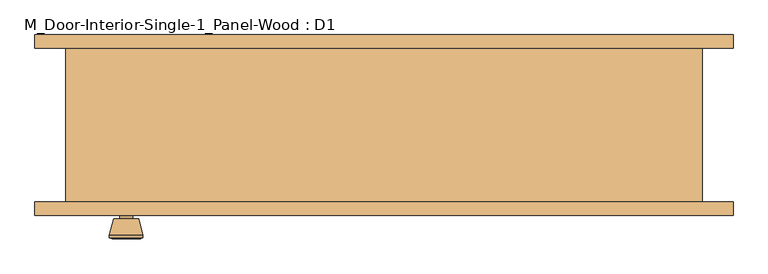
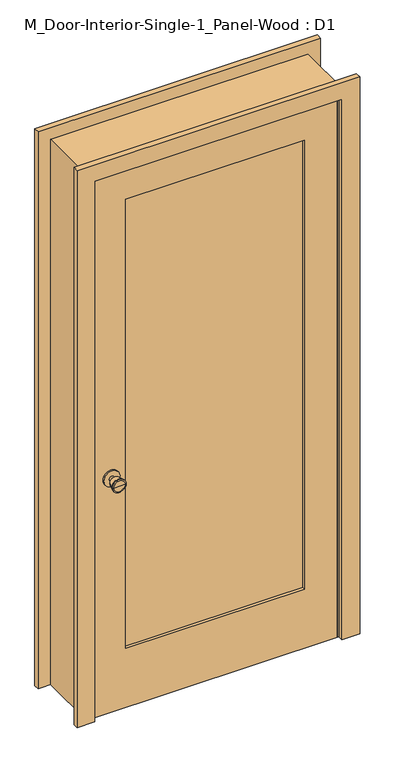
"""IFC4 building model written with IfcOpenShell, lengths in millimetres: door geometry, M_Door-Interior-Single-1_Panel-Wood : D1."""

from ifc_helpers import new_model, si_unit, point, frame, frame_2d, origin, place, context, project, spatial, polyline, circle_curve, trimmed, segment, composite_curve, outline, extrude, faceted_brep, source, transform, mapped, element, save
from ifc_brep_helpers import plane_surface, cylinder_surface, revolved_surface, advanced_brep


def m_door_interior_single_1_panel_wood_d1_ac8a812a(model_context):
    return source(origin(), model_context, "Body", "SolidModel", [
        advanced_brep(
        [(-385.0, -70.825, 914.4), (-395.0, -70.825, 914.4), (-375.0, -70.825, 914.4), (-364.5241324, -21.825, 914.4), (-405.4758676, -21.825, 914.4), (-385.0, -21.825, 914.4), (-360.0, -23.6528681, 914.4), (-410.0, -23.6528681, 914.4), (-360.0, -27.1165463, 914.4), (-410.0, -27.1165463, 914.4), (-366.363764, -51.825, 914.4), (-403.636236, -51.825, 914.4), (-375.0, -51.825, 914.4), (-395.0, -51.825, 914.4)],
        [
            (0, 1),
            (1, 2, circle_curve(frame((-385.0, -70.825, 914.4), z_axis=(0.0, -1.0, 0.0), x_axis=(-1.0, 0.0, 0.0)), 10.0)),
            (2, 0),
            (2, 1, circle_curve(frame((-385.0, -70.825, 914.4), z_axis=(0.0, -1.0, 0.0), x_axis=(-1.0, 0.0, 0.0)), 10.0)),
            (3, 4, circle_curve(frame((-385.0, -21.825, 914.4), z_axis=(0.0, 1.0, 0.0), x_axis=(-1.0, 0.0, 0.0)), 20.4758676)),
            (4, 5),
            (5, 3),
            (4, 3, circle_curve(frame((-385.0, -21.825, 914.4), z_axis=(0.0, 1.0, 0.0), x_axis=(-1.0, 0.0, 0.0)), 20.4758676)),
            (6, 7, circle_curve(frame((-385.0, -23.6528681, 914.4), z_axis=(0.0, 1.0, 0.0), x_axis=(-1.0, 0.0, 0.0)), 25.0)),
            (7, 4),
            (3, 6),
            (7, 6, circle_curve(frame((-385.0, -23.6528681, 914.4), z_axis=(0.0, 1.0, 0.0), x_axis=(-1.0, 0.0, 0.0)), 25.0)),
            (8, 9, circle_curve(frame((-385.0, -27.1165463, 914.4), z_axis=(0.0, 1.0, 0.0), x_axis=(-1.0, 0.0, 0.0)), 25.0)),
            (9, 7),
            (6, 8),
            (9, 8, circle_curve(frame((-385.0, -27.1165463, 914.4), z_axis=(0.0, 1.0, 0.0), x_axis=(-1.0, 0.0, 0.0)), 25.0)),
            (10, 11, circle_curve(frame((-385.0, -51.825, 914.4), z_axis=(0.0, 1.0, 0.0), x_axis=(-1.0, 0.0, 0.0)), 18.636236)),
            (11, 9),
            (8, 10),
            (11, 10, circle_curve(frame((-385.0, -51.825, 914.4), z_axis=(0.0, 1.0, 0.0), x_axis=(-1.0, 0.0, 0.0)), 18.636236)),
            (12, 13, circle_curve(frame((-385.0, -51.825, 914.4), z_axis=(0.0, 1.0, 0.0), x_axis=(-1.0, 0.0, 0.0)), 10.0)),
            (13, 11),
            (10, 12),
            (13, 12, circle_curve(frame((-385.0, -51.825, 914.4), z_axis=(0.0, 1.0, 0.0), x_axis=(-1.0, 0.0, 0.0)), 10.0)),
            (1, 13),
            (12, 2),
        ],
        [
            plane_surface(frame((-385.0, -70.825, 914.4), z_axis=(0.0, -1.0, 0.0), x_axis=(-1.0, 0.0, 0.0))),
            plane_surface(frame((-385.0, -21.825, 914.4), z_axis=(0.0, 1.0, 0.0), x_axis=(-1.0, 0.0, 0.0))),
            revolved_surface(polyline([(-405.4758676, -21.825, 914.4), (-410.0, -23.6528681, 914.4)]), (-385.0, -70.825, 914.4), (0.0, -1.0, 0.0)),
            cylinder_surface(frame((-385.0, -70.825, 914.4), z_axis=(0.0, -1.0, 0.0), x_axis=(-1.0, 0.0, 0.0)), 25.0),
            revolved_surface(polyline([(-410.0, -27.1165463, 914.4), (-403.636236, -51.825, 914.4)]), (-385.0, -70.825, 914.4), (0.0, -1.0, 0.0)),
            plane_surface(frame((-385.0, -51.825, 914.4), z_axis=(0.0, -1.0, 0.0), x_axis=(-1.0, 0.0, 0.0))),
            cylinder_surface(frame((-385.0, -70.825, 914.4), z_axis=(0.0, -1.0, 0.0), x_axis=(-1.0, 0.0, 0.0)), 10.0),
        ],
        [
            (0, [[1, 2, 3]]),
            (0, [[-3, 4, -1]]),
            (1, [[5, 6, 7]]),
            (1, [[8, -7, -6]]),
            (2, [[9, 10, -5, 11]]),
            (2, [[12, -11, -8, -10]]),
            (3, [[13, 14, -9, 15]]),
            (3, [[16, -15, -12, -14]]),
            (4, [[17, 18, -13, 19]]),
            (4, [[20, -19, -16, -18]]),
            (5, [[21, 22, -17, 23]]),
            (5, [[24, -23, -20, -22]]),
            (6, [[-2, 25, -21, 26]]),
            (6, [[-4, -26, -24, -25]]),
        ],
    ),
        extrude(outline(composite_curve([segment(trimmed(circle_curve(frame_2d((914.4, -385.0)), 30.0), [point((914.4, -415.0))], [point((914.4, -355.0))], False, "CARTESIAN"), True, "CONTINUOUS"), segment(trimmed(circle_curve(frame_2d((914.4, -385.0)), 30.0), [point((914.4, -355.0))], [point((914.4, -415.0))], False, "CARTESIAN"), True, "CONTINUOUS")], self_intersect=False)), frame((0.0, -76.825, 0.0), z_axis=(0.0, 1.0, 0.0), x_axis=(0.0, 0.0, 1.0)), (0.0, 0.0, 1.0), 6.0),
        advanced_brep(
        [(-385.0, -117.825, 914.4), (-375.0, -117.825, 914.4), (-395.0, -117.825, 914.4), (-364.5241324, -166.825, 914.4), (-385.0, -166.825, 914.4), (-405.4758676, -166.825, 914.4), (-360.0, -164.9971319, 914.4), (-410.0, -164.9971319, 914.4), (-360.0, -161.5334537, 914.4), (-410.0, -161.5334537, 914.4), (-366.363764, -136.825, 914.4), (-403.636236, -136.825, 914.4), (-375.0, -136.825, 914.4), (-395.0, -136.825, 914.4)],
        [
            (0, 1),
            (1, 2, circle_curve(frame((-385.0, -117.825, 914.4), z_axis=(0.0, 1.0, 0.0), x_axis=(-1.0, 0.0, 0.0)), 10.0)),
            (2, 0),
            (2, 1, circle_curve(frame((-385.0, -117.825, 914.4), z_axis=(0.0, 1.0, 0.0), x_axis=(-1.0, 0.0, 0.0)), 10.0)),
            (3, 4),
            (4, 5),
            (5, 3, circle_curve(frame((-385.0, -166.825, 914.4), z_axis=(0.0, -1.0, 0.0), x_axis=(-1.0, 0.0, 0.0)), 20.4758676)),
            (3, 5, circle_curve(frame((-385.0, -166.825, 914.4), z_axis=(0.0, -1.0, 0.0), x_axis=(-1.0, 0.0, 0.0)), 20.4758676)),
            (6, 3),
            (5, 7),
            (7, 6, circle_curve(frame((-385.0, -164.9971319, 914.4), z_axis=(0.0, -1.0, 0.0), x_axis=(-1.0, 0.0, 0.0)), 25.0)),
            (6, 7, circle_curve(frame((-385.0, -164.9971319, 914.4), z_axis=(0.0, -1.0, 0.0), x_axis=(-1.0, 0.0, 0.0)), 25.0)),
            (8, 6),
            (7, 9),
            (9, 8, circle_curve(frame((-385.0, -161.5334537, 914.4), z_axis=(0.0, -1.0, 0.0), x_axis=(-1.0, 0.0, 0.0)), 25.0)),
            (8, 9, circle_curve(frame((-385.0, -161.5334537, 914.4), z_axis=(0.0, -1.0, 0.0), x_axis=(-1.0, 0.0, 0.0)), 25.0)),
            (10, 8),
            (9, 11),
            (11, 10, circle_curve(frame((-385.0, -136.825, 914.4), z_axis=(0.0, -1.0, 0.0), x_axis=(-1.0, 0.0, 0.0)), 18.636236)),
            (10, 11, circle_curve(frame((-385.0, -136.825, 914.4), z_axis=(0.0, -1.0, 0.0), x_axis=(-1.0, 0.0, 0.0)), 18.636236)),
            (12, 10),
            (11, 13),
            (13, 12, circle_curve(frame((-385.0, -136.825, 914.4), z_axis=(0.0, -1.0, 0.0), x_axis=(-1.0, 0.0, 0.0)), 10.0)),
            (12, 13, circle_curve(frame((-385.0, -136.825, 914.4), z_axis=(0.0, -1.0, 0.0), x_axis=(-1.0, 0.0, 0.0)), 10.0)),
            (1, 12),
            (13, 2),
        ],
        [
            plane_surface(frame((-385.0, -117.825, 914.4), z_axis=(0.0, 1.0, 0.0), x_axis=(-1.0, 0.0, 0.0))),
            plane_surface(frame((-385.0, -166.825, 914.4), z_axis=(0.0, -1.0, 0.0), x_axis=(-1.0, 0.0, 0.0))),
            revolved_surface(polyline([(-405.4758676, -166.825, 914.4), (-410.0, -164.9971319, 914.4)]), (-385.0, -117.825, 914.4), (0.0, 1.0, 0.0)),
            cylinder_surface(frame((-385.0, -117.825, 914.4), z_axis=(0.0, 1.0, 0.0), x_axis=(-1.0, 0.0, 0.0)), 25.0),
            revolved_surface(polyline([(-410.0, -161.5334537, 914.4), (-403.636236, -136.825, 914.4)]), (-385.0, -117.825, 914.4), (0.0, 1.0, 0.0)),
            plane_surface(frame((-385.0, -136.825, 914.4), z_axis=(0.0, 1.0, 0.0), x_axis=(-1.0, 0.0, 0.0))),
            cylinder_surface(frame((-385.0, -117.825, 914.4), z_axis=(0.0, 1.0, 0.0), x_axis=(-1.0, 0.0, 0.0)), 10.0),
        ],
        [
            (0, [[1, 2, 3]]),
            (0, [[-3, 4, -1]]),
            (1, [[5, 6, 7]]),
            (1, [[-6, -5, 8]]),
            (2, [[9, -7, 10, 11]]),
            (2, [[-10, -8, -9, 12]]),
            (3, [[13, -11, 14, 15]]),
            (3, [[-14, -12, -13, 16]]),
            (4, [[17, -15, 18, 19]]),
            (4, [[-18, -16, -17, 20]]),
            (5, [[21, -19, 22, 23]]),
            (5, [[-22, -20, -21, 24]]),
            (6, [[25, -23, 26, -2]]),
            (6, [[-26, -24, -25, -4]]),
        ],
    ),
        extrude(outline(composite_curve([segment(trimmed(circle_curve(frame_2d((914.4, -385.0)), 30.0), [point((914.4, -415.0))], [point((914.4, -355.0))], False, "CARTESIAN"), True, "CONTINUOUS"), segment(trimmed(circle_curve(frame_2d((914.4, -385.0)), 30.0), [point((914.4, -355.0))], [point((914.4, -415.0))], False, "CARTESIAN"), True, "CONTINUOUS")], self_intersect=False)), frame((0.0, -117.825, 0.0), z_axis=(0.0, 1.0, 0.0), x_axis=(0.0, 0.0, 1.0)), (0.0, 0.0, 1.0), 6.0),
        extrude(outline(polyline([(330.0, -88.4916667), (330.0, -100.1583333), (-330.0, -100.1583333), (-330.0, -88.4916667), (330.0, -88.4916667)])), frame((0.0, 0.0, 230.0), z_axis=(0.0, 0.0, 1.0), x_axis=(1.0, 0.0, 0.0)), (0.0, 0.0, 1.0), 1750.0),
        extrude(outline(polyline([(2100.0, -450.0), (0.0, -450.0), (0.0, 450.0), (2100.0, 450.0), (2100.0, -450.0)]), holes=[polyline([(1980.0, -330.0), (1980.0, 330.0), (230.0, 330.0), (230.0, -330.0), (1980.0, -330.0)])]), frame((0.0, -111.825, 0.0), z_axis=(0.0, 1.0, 0.0), x_axis=(0.0, 0.0, 1.0)), (0.0, 0.0, 1.0), 35.0),
        faceted_brep([(475.0, -111.825, 0.0), (450.0, -111.825, 0.0), (450.0, -76.825, 0.0), (437.3, -76.825, 0.0), (437.3, -41.9, 0.0), (450.0, -41.9, 0.0), (450.0, 118.175, 0.0), (475.0, 118.175, 0.0), (475.0, 118.175, 2125.0), (475.0, -111.825, 2125.0), (450.0, 118.175, 2100.0), (-450.0, 118.175, 2100.0), (-450.0, 118.175, 0.0), (-475.0, 118.175, 0.0), (-475.0, 118.175, 2125.0), (450.0, -41.9, 2100.0), (437.3, -41.9, 2087.3), (-437.3, -41.9, 2087.3), (-437.3, -41.9, 0.0), (-450.0, -41.9, 0.0), (-450.0, -41.9, 2100.0), (437.3, -76.825, 2087.3), (450.0, -76.825, 2100.0), (-450.0, -76.825, 2100.0), (-450.0, -76.825, 0.0), (-437.3, -76.825, 0.0), (-437.3, -76.825, 2087.3), (450.0, -111.825, 2100.0), (-475.0, -111.825, 2125.0), (-475.0, -111.825, 0.0), (-450.0, -111.825, 0.0), (-450.0, -111.825, 2100.0)], [[[0, 1, 2, 3, 4, 5, 6, 7]], [[7, 8, 9, 0]], [[6, 10, 11, 12, 13, 14, 8, 7]], [[5, 15, 10, 6]], [[4, 16, 17, 18, 19, 20, 15, 5]], [[3, 21, 16, 4]], [[2, 22, 23, 24, 25, 26, 21, 3]], [[1, 27, 22, 2]], [[0, 9, 28, 29, 30, 31, 27, 1]], [[8, 14, 28, 9]], [[15, 20, 11, 10]], [[21, 26, 17, 16]], [[27, 31, 23, 22]], [[29, 13, 12, 19, 18, 25, 24, 30]], [[14, 13, 29, 28]], [[20, 19, 12, 11]], [[26, 25, 18, 17]], [[31, 30, 24, 23]]]),
        extrude(outline(polyline([(0.0, 521.35), (2171.35, 521.35), (2171.35, -521.35), (0.0, -521.35), (0.0, -456.35), (2106.35, -456.35), (2106.35, 456.35), (0.0, 456.35), (0.0, 521.35)])), frame((0.0, 118.175, 0.0), z_axis=(0.0, 1.0, 0.0), x_axis=(0.0, 0.0, 1.0)), (0.0, 0.0, 1.0), 20.0),
        extrude(outline(polyline([(0.0, 521.35), (2171.35, 521.35), (2171.35, -521.35), (0.0, -521.35), (0.0, -456.35), (2106.35, -456.35), (2106.35, 456.35), (0.0, 456.35), (0.0, 521.35)])), frame((0.0, -131.825, 0.0), z_axis=(0.0, 1.0, 0.0), x_axis=(0.0, 0.0, 1.0)), (0.0, 0.0, 1.0), 20.0),
    ])


if __name__ == "__main__":
    model = new_model("IFC4")
    model_context = context("Model", 3, world=origin())
    ifc_project = project(units=[si_unit("LENGTHUNIT", "METRE", prefix="MILLI")], contexts=[model_context])
    site = spatial("IfcSite", under=ifc_project)
    building = spatial("IfcBuilding", under=site)
    placement = place(None, origin())
    m_door_interior_single_1_panel_wood_d1_shape = m_door_interior_single_1_panel_wood_d1_ac8a812a(model_context)
    element("IfcDoor", 1, ObjectType="M_Door-Interior-Single-1_Panel-Wood : D1", at=placement, inside=building, context=model_context, shape_type="MappedRepresentation", body=[
        mapped(m_door_interior_single_1_panel_wood_d1_shape, transform((0.0, 0.0, 0.0), x_axis=(1.0, 0.0, 0.0), y_axis=(0.0, 1.0, 0.0), z_axis=(0.0, 0.0, 1.0))),
    ])
    save(model, "model.ifc")

# Revit data of these elements
# Type "M_Door-Interior-Single-1_Panel-Wood : D1"
#   Type Mark = "49"
#   Assembly Code = "C1020300"
#   Analytic Construction = "Wooden"
#   Top Rail = 12 cm
#   Thickness = 3.5 cm
#   Thermal Resistance (R) = 0.455703 (m²·K)/W
#   Swing Angle [instance default] = 90.00°
#   Stiles = 12 cm
#   Rough Width = 95 cm
#   Rough Height = 212.5 cm
#   Height = 210 cm
#   Width = 90 cm
#   Heat Transfer Coefficient (U) = 2.19465 W/(m²·K)
#   Bottom Rail = 23 cm
#   Trim Material = Cherry
#   Panel Material = Cherry
#   Frame Material = Cherry
#   Door Handle Material = Aluminum
#   Visual Light Transmittance = 0
#   Solar Heat Gain Coefficient = 0
#   Wall Closure = (empty or 0)
#   Function = (empty or 0)
# Element 1 (IfcDoor, "M_Door-Interior-Single-1_Panel-Wood : D1")
#   Materials on its faces: "Cherry", "Aluminum"
# Materials
#   "Cherry": class "Wood", colour RGB 226 177 128, transparency 0, Description = "Prunus Serotina", Cost = 0
#   "Aluminum": class "Metal", colour RGB 247 247 247, transparency 0, Description = "Aluminum 6061", Cost = 0
